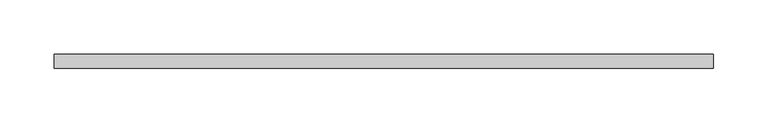
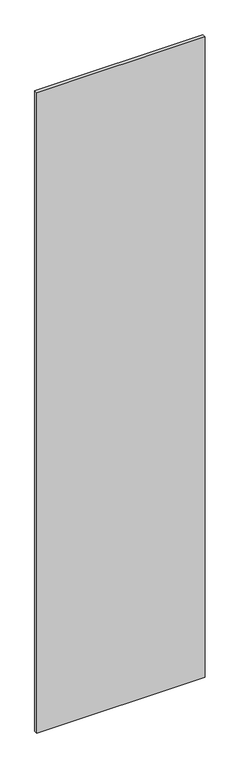
"""IFC4 building model written with IfcOpenShell, lengths in millimetres: proxy geometry, Inner panel:Inner panel:1:Inner panel:1 : Inner panel:Inner panel:300324:300043:Inner panel:1:Inner panel:1 : Inner panel:Inner panel:300324:300043 : Inner panel:Inner panel:1:Inner panel:1 : Inner panel:Inner panel:300324:300043:27 : Inner panel:Inner panel:1:Inner panel:1 : Inner panel:Inner panel:300324:300043:Inner panel:1:Inner panel:1 : Inner panel:Inner panel:300324:300043 : Inner panel:Inner panel:1:Inner panel:1 : Inner panel:Inner panel:300324:300043:300031."""

from ifc_helpers import new_model, si_unit, frame, origin, place, context, project, spatial, polyline, outline, extrude, source, transform, mapped, element, save


def generic_models_c0582be2(model_context):
    return source(origin(), model_context, "Body", "SweptSolid", [
        extrude(outline(polyline([(593738.0867239, -579000.6913841), (594344.5117239, -579000.6913841), (594344.5117239, -579013.3913841), (593738.0867239, -579013.3913841), (593738.0867239, -579000.6913841)])), frame((0.0, 0.0, 1270.0), z_axis=(0.0, 0.0, 1.0), x_axis=(1.0, 0.0, 0.0)), (0.0, 0.0, 1.0), 2438.4),
    ])


if __name__ == "__main__":
    model = new_model("IFC4")
    model_context = context("Model", 3, world=origin())
    ifc_project = project(units=[si_unit("LENGTHUNIT", "METRE", prefix="MILLI")], contexts=[model_context])
    site = spatial("IfcSite", under=ifc_project)
    building = spatial("IfcBuilding", under=site)
    placement = place(None, origin())
    generic_models_shape = generic_models_c0582be2(model_context)
    element("IfcBuildingElementProxy", 1, Name="Inner panel:Inner panel:1:Inner panel:1 : Inner panel:Inner panel:300324:300043:Inner panel:1:Inner panel:1 : Inner panel:Inner panel:300324:300043 : Inner panel:Inner panel:1:Inner panel:1 : Inner panel:Inner panel:300324:300043:27 : Inner panel:Inner panel:1:Inner panel:1 : Inner panel:Inner panel:300324:300043:Inner panel:1:Inner panel:1 : Inner panel:Inner panel:300324:300043 : Inner panel:Inner panel:1:Inner panel:1 : Inner panel:Inner panel:300324:300043:300031", ObjectType="Inner panel:Inner panel:1:Inner panel:1 : Inner panel:Inner panel:300324:300043:Inner panel:1:Inner panel:1 : Inner panel:Inner panel:300324:300043 : Inner panel:Inner panel:1:Inner panel:1 : Inner panel:Inner panel:300324:300043:27 : Inner panel:Inner panel:1:Inner panel:1 : Inner panel:Inner panel:300324:300043:Inner panel:1:Inner panel:1 : Inner panel:Inner panel:300324:300043 : Inner panel:Inner panel:1:Inner panel:1 : Inner panel:Inner panel:300324:300043:300031", at=placement, inside=building, context=model_context, shape_type="MappedRepresentation", body=[
        mapped(generic_models_shape, transform((0.0, 0.0, 0.0), x_axis=(1.0, 0.0, 0.0), y_axis=(0.0, 1.0, 0.0), z_axis=(0.0, 0.0, 1.0))),
    ])
    save(model, "model.ifc")

# Revit data of these elements
# Type "Inner panel:Inner panel:1:Inner panel:1 : Inner panel:Inner panel:300324:300043:Inner panel:1:Inner panel:1 : Inner panel:Inner panel:300324:300043 : Inner panel:Inner panel:1:Inner panel:1 : Inner panel:Inner panel:300324:300043:27 : Inner panel:Inner panel:1:Inner panel:1 : Inner panel:Inner panel:300324:300043:Inner panel:1:Inner panel:1 : Inner panel:Inner panel:300324:300043 : Inner panel:Inner panel:1:Inner panel:1 : Inner panel:Inner panel:300324:300043:300031"
#   NameOverride = "Inner panel:Inner panel:1:Inner panel:1 : Inner panel:Inner panel:300324:300043:Inner panel:1:Inner panel:1 : Inner panel:Inner panel:300324:300043 : Inner panel:Inner panel:1:Inner panel:1 : Inner panel:Inner panel:300324:300043:300031"
#   ObjectTypeOverride = "Inner panel:1:Inner panel:1 : Inner panel:Inner panel:300324:300043 : Inner panel:Inner panel:1:Inner panel:1 : Inner panel:Inner panel:300324:300043"
#   Reference = "Inner panel"
#   Tag = "300031"
# Element 1 (IfcBuildingElementProxy, "Inner panel:Inner panel:1:Inner panel:1 : Inner panel:Inner panel:300324:300043:Inner panel:1:Inner panel:1 : Inner panel:Inner panel:300324:300043 : Inner panel:Inner panel:1:Inner panel:1 : Inner panel:Inner panel:300324:300043:27 : Inner panel:Inner panel:1:Inner panel:1 : Inner panel:Inner panel:300324:300043:Inner panel:1:Inner panel:1 : Inner panel:Inner panel:300324:300043 : Inner panel:Inner panel:1:Inner panel:1 : Inner panel:Inner panel:300324:300043:300031")
#   Materials on its faces: "1/2\" FIBERGLASS MAT GYPSUM PANELS"
# Materials
#   "1/2\" FIBERGLASS MAT GYPSUM PANELS": class "Generic", colour RGB 171 170 168, transparency 0, Description = "Gypsum Wall Board", Cost = 0
